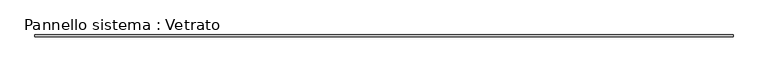
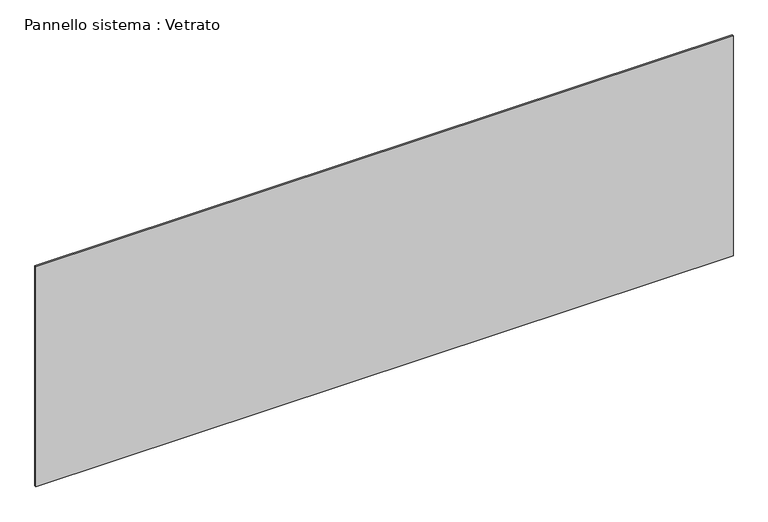
"""IFC4 building model written with IfcOpenShell, lengths in millimetres: plate geometry, Pannello sistema : Vetrato."""

from ifc_helpers import new_model, si_unit, origin, origin_with_axes, place, context, project, spatial, polyline, outline, extrude, source, transform, mapped, element, save


def pannello_sistema_vetrato_3a8c62e0(model_context):
    return source(origin(), model_context, "Body", "SweptSolid", [
        extrude(outline(polyline([(6000.0, -15.0), (-6000.0, -15.0), (-6000.0, 15.0), (6000.0, 15.0), (6000.0, -15.0)])), origin_with_axes(), (0.0, 0.0, 1.0), 4000.0),
    ])


if __name__ == "__main__":
    model = new_model("IFC4")
    model_context = context("Model", 3, world=origin())
    ifc_project = project(units=[si_unit("LENGTHUNIT", "METRE", prefix="MILLI")], contexts=[model_context])
    site = spatial("IfcSite", under=ifc_project)
    building = spatial("IfcBuilding", under=site)
    placement = place(None, origin())
    pannello_sistema_vetrato_shape = pannello_sistema_vetrato_3a8c62e0(model_context)
    element("IfcPlate", 1, ObjectType="Pannello sistema : Vetrato", at=placement, inside=building, context=model_context, shape_type="MappedRepresentation", body=[
        mapped(pannello_sistema_vetrato_shape, transform((0.0, 0.0, 0.0), x_axis=(1.0, 0.0, 0.0), y_axis=(0.0, 1.0, 0.0), z_axis=(0.0, 0.0, 1.0))),
    ])
    save(model, "model.ifc")

# Revit data of these elements
# Type "Pannello sistema : Vetrato"
#   Construction Type Id = "GSP4R"
#   Analytic Construction = "Vetrata singola Pilkington 1/8 in"
#   Visual Light Transmittance = 0.9
#   Solar Heat Gain Coefficient = 0.86
#   Heat Transfer Coefficient (U) = 6.7069 W/(m²·K)
# Element 1 (IfcPlate, "Pannello sistema : Vetrato")
#   Materials on its faces: "Default - Vetro"
# Materials
#   "Default - Vetro": class "Vetro", colour RGB 208 208 208, transparency 0.7, Cost = 0
